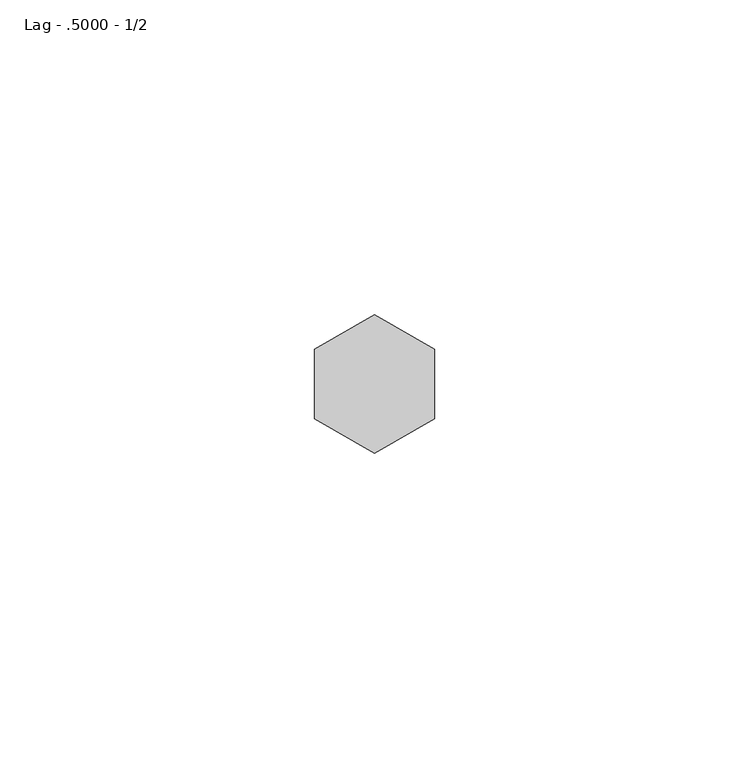
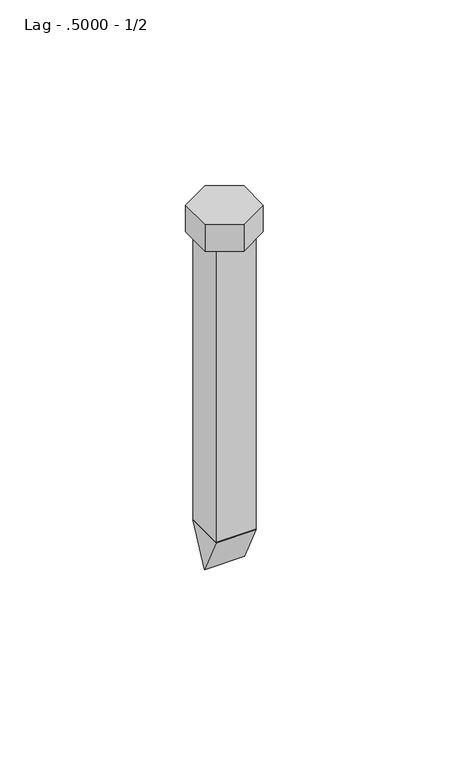
"""IFC4 building model written with IfcOpenShell, lengths in millimetres: fastener geometry, 060523 - W_P_C - Fastenings - Generic - SQUARE : Lag - .5000 - 1/2."""

from ifc_helpers import new_model, si_unit, frame, origin, origin_with_axes, place, context, project, spatial, polyline, outline, extrude, source, transform, mapped, element, save


def lag_5000_1_2_34a09ce3(model_context):
    return source(origin(), model_context, "Body", "SweptSolid", [
        extrude(outline(polyline([(0.0, -114.696875), (-6.5484375, -101.6), (6.5484375, -101.6), (0.0, -114.696875)])), frame((-6.5484375, 0.0, 0.0), z_axis=(1.0, 0.0, 0.0), x_axis=(0.0, 1.0, 0.0)), (0.0, 0.0, 1.0), 13.096875),
        extrude(outline(polyline([(-9.525, 5.4992613), (0.0, 10.9985226), (9.525, 5.4992613), (9.525, -5.4992613), (0.0, -10.9985226), (-9.525, -5.4992613), (-9.525, 5.4992613)])), origin_with_axes(), (0.0, 0.0, 1.0), 9.2273437),
        extrude(outline(polyline([(-6.5484375, 6.5484375), (6.5484375, 6.5484375), (6.5484375, -6.5484375), (-6.5484375, -6.5484375), (-6.5484375, 6.5484375)])), frame((0.0, 0.0, -101.6), z_axis=(0.0, 0.0, 1.0), x_axis=(1.0, 0.0, 0.0)), (0.0, 0.0, 1.0), 101.6),
    ])


if __name__ == "__main__":
    model = new_model("IFC4")
    model_context = context("Model", 3, world=origin())
    ifc_project = project(units=[si_unit("LENGTHUNIT", "METRE", prefix="MILLI")], contexts=[model_context])
    site = spatial("IfcSite", under=ifc_project)
    building = spatial("IfcBuilding", under=site)
    placement = place(None, origin())
    lag_5000_1_2_shape = lag_5000_1_2_34a09ce3(model_context)
    element("IfcFastener", 1, ObjectType="060523 - W_P_C - Fastenings - Generic - SQUARE : Lag - .5000 - 1/2", at=placement, inside=building, context=model_context, shape_type="MappedRepresentation", body=[
        mapped(lag_5000_1_2_shape, transform((0.0, 0.0, 0.0), x_axis=(1.0, 0.0, 0.0), y_axis=(0.0, 1.0, 0.0), z_axis=(0.0, 0.0, 1.0))),
    ])
    save(model, "model.ifc")

# Revit data of these elements
# Type "060523 - W_P_C - Fastenings - Generic - SQUARE : Lag - .5000 - 1/2"
#   Washer_Thickness = 0' - 0 31/256"
#   Washer Radius = 0' - 0 159/256"
#   Washer Offset - Head = 0' - 0"
#   Washer Offset = 0' - 0"
#   Thickness_of_Substrate [instance default] = 0' - 1"
#   Side = 0' - 0 111/256"
#   Radius = 0' - 0 33/128"
#   Length [instance default] = 0' - 4"
#   Head Size = 0' - 0 3/4"
#   Head Radius = 0' - 0 3/8"
#   Head Height = 0' - 0 93/256"
#   Double Diameter = 0' - 1 1/32"
#   Diameter = 0' - 0 33/64"
#   Default Elevation = 4' - 0"
#   Washer_Nut_Visibility = no
#   Washer_Head_Visibility = no
#   Round_Head_Visibility = no
#   Point Visibility = yes
#   Nut_Visibility = no
#   Hex_Head_Visiblilty = yes
#   Washer Material = none
#   Bolt Material (Size) = AT SILL - FASTENER AT 24" O.C.
# Element 1 (IfcFastener, "060523 - W_P_C - Fastenings - Generic - SQUARE : Lag - .5000 - 1/2")
#   Materials on its faces: "AT SILL - FASTENER AT 24\" O.C."
# Materials
#   "AT SILL - FASTENER AT 24\" O.C.": class "Generic", colour RGB 120 120 120, transparency 0, Cost = 0
